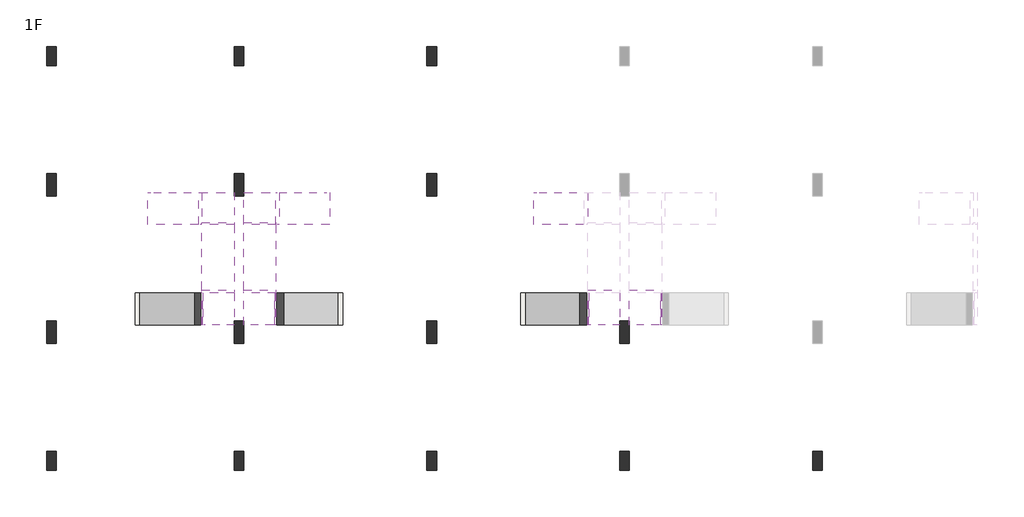
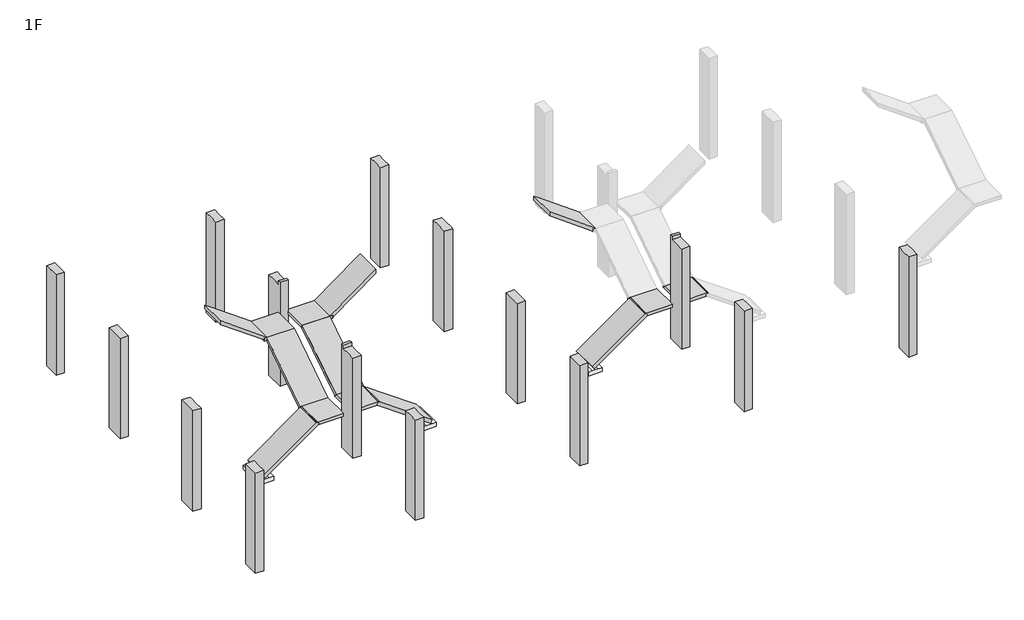
# One storey, part 1 of 2: 15 columns, 14 beams, 3 slabs.
"""IFC4 building model written with IfcOpenShell, lengths in millimetres."""

from ifc_helpers import new_model, si_unit, frame, origin, place, context, project, spatial, polyline, outline, extrude, faceted_brep, element, save

model = new_model("IFC4")

# Units and contexts
model_context = context("Model", 3, world=origin())
ifc_project = project(units=[si_unit("LENGTHUNIT", "METRE", prefix="MILLI")], contexts=[model_context])

# Site, building, storey
site = spatial("IfcSite", under=ifc_project)
building = spatial("IfcBuilding", under=site)
storey = spatial("IfcBuildingStorey", under=building, Name="1F", Elevation=30.0)

# Beams
placement = place(None, origin())
element("IfcBeam", 1, ObjectType="M_Concrete-Rectangular Beam : 1000x120", at=placement, inside=storey, context=model_context, shape_type="Brep", body=[
    faceted_brep([(4730.4772067, 5424.9999998, 1421.3386706), (4730.4772067, 4424.9999998, 1421.3386706), (4730.7175592, 4424.9999998, 1421.0), (4799.9279185, 4424.9999998, 1323.4785734), (4799.9279185, 5424.9999998, 1323.4785734), (4730.7175592, 5424.9999998, 1421.0), (2770.0, 5424.9999998, 30.0), (2839.4507118, 5424.9999998, -67.8600972), (2839.4507118, 4424.9999998, -67.8600972), (2770.0, 4424.9999998, 30.0), (4730.0, 5424.9999998, 1421.0), (4700.0000007, 5424.9999998, 1399.7091842), (4700.0000007, 4424.9999998, 1399.7091842), (4730.0, 4424.9999998, 1421.0), (4768.2542996, 4424.9999998, 1301.0), (4768.2542996, 5424.9999998, 1301.0)], [[[0, 1, 2, 3, 4, 5]], [[6, 7, 8, 9]], [[1, 0, 10, 11, 6, 9, 12, 13]], [[3, 2, 1, 13, 12, 9, 8, 14]], [[4, 3, 14, 8, 7, 15]], [[0, 5, 4, 15, 7, 6, 11, 10]]]),
])
element("IfcBeam", 2, ObjectType="M_Concrete-Rectangular Beam : 1000x120", at=placement, inside=storey, context=model_context, shape_type="Brep", body=[
    faceted_brep([(4700.0000007, 7550.0000002, 2813.0), (5700.0000007, 7550.0000002, 2813.0), (5700.0000007, 7615.755173, 2712.6194379), (4700.0000007, 7615.755173, 2712.6194379), (4700.0000007, 5424.9999998, 1421.0), (4700.0000007, 5490.7551727, 1320.6194379), (5700.0000007, 5490.7551727, 1320.6194379), (5700.0000007, 5424.9999998, 1421.0), (5700.0000007, 5524.9999998, 1343.0518141), (5700.0000007, 7585.8045224, 2693.0), (4700.0000007, 5524.9999998, 1343.0518141), (4700.0000007, 7585.8045224, 2693.0)], [[[0, 1, 2, 3]], [[4, 5, 6, 7]], [[1, 0, 4, 7]], [[2, 1, 7, 6, 8, 9]], [[3, 2, 9, 8, 6, 5, 10, 11]], [[0, 3, 11, 10, 5, 4]]]),
])
element("IfcBeam", 3, ObjectType="M_Concrete-Rectangular Beam : 1000x120", at=placement, inside=storey, context=model_context, shape_type="Brep", body=[
    faceted_brep([(4600.0000007, 7550.0000002, 2813.0), (4600.0000007, 8550.0000002, 2813.0), (4600.0000007, 8550.0000002, 2693.0), (4600.0000007, 7550.0000002, 2693.0), (5700.0000007, 8550.0000002, 2693.0), (5700.0000007, 8550.0000002, 2813.0), (5700.0000007, 7550.0000002, 2813.0), (5700.0000007, 7615.755173, 2712.6194379), (5700.0000007, 7585.8045224, 2693.0), (4700.0000007, 7550.0000002, 2813.0), (4700.0000007, 7585.8045224, 2693.0), (4700.0000007, 7550.0000002, 2693.0), (4700.0000007, 7615.755173, 2712.6194379)], [[[0, 1, 2, 3]], [[4, 5, 6, 7, 8]], [[1, 0, 9, 6, 5]], [[2, 1, 5, 4]], [[3, 2, 4, 8, 10, 11]], [[0, 3, 11, 9]], [[12, 7, 6, 9]], [[7, 12, 10, 8]], [[12, 9, 11, 10]]]),
])
element("IfcBeam", 4, ObjectType="M_Concrete-Rectangular Beam : 1000x120", at=placement, inside=storey, context=model_context, shape_type="Brep", body=[
    faceted_brep([(3020.0, 8549.9999993, 4029.9999711), (3020.0, 7549.9999993, 4029.9999711), (4699.9999533, 7549.9999993, 2813.0), (4699.9999533, 8549.9999993, 2813.0), (3199.4576422, 8549.9999993, 3900.0), (4600.0000007, 8549.9999993, 2813.0), (4600.0000007, 8549.9999993, 2737.262925), (3020.0, 8549.9999993, 3881.8224539), (3020.0, 8549.9999993, 3900.0), (3020.0, 7549.9999993, 3881.8224539), (4600.0000007, 7549.9999993, 2737.262925), (4600.0000007, 7549.9999993, 2813.0), (3020.0, 7549.9999993, 3900.0)], [[[0, 1, 2, 3, 4]], [[5, 6, 7, 8, 0, 4, 3]], [[9, 7, 6, 10]], [[10, 11, 2, 1, 12, 9]], [[1, 0, 8, 7, 9, 12]], [[5, 11, 10, 6]], [[11, 5, 3, 2]]]),
])
element("IfcBeam", 5, ObjectType="M_Concrete-Rectangular Beam : 1000x120", at=placement, inside=storey, context=model_context, shape_type="Brep", body=[
    faceted_brep([(5700.0000007, 5524.9999998, 1301.0), (4700.0000007, 5524.9999998, 1301.0), (4700.0000007, 5524.9999998, 1343.0518141), (5700.0000007, 5524.9999998, 1343.0518141), (5700.0000007, 4424.9999998, 1301.0), (5700.0000007, 4424.9999998, 1421.0), (4730.7175592, 4424.9999998, 1421.0), (4799.9279185, 4424.9999998, 1323.4785734), (4768.2542996, 4424.9999998, 1301.0), (4730.0, 4424.9999998, 1421.0), (4730.0, 5424.9999998, 1421.0), (4700.0000007, 5424.9999998, 1421.0), (4700.0000007, 4424.9999998, 1421.0), (5700.0000007, 5490.7551727, 1320.6194379), (5700.0000007, 5424.9999998, 1421.0), (4768.2542996, 5424.9999998, 1301.0), (4700.0000007, 5424.9999998, 1301.0), (4700.0000007, 5424.9999998, 1399.7091842), (4700.0000007, 4424.9999998, 1399.7091842), (4700.0000007, 5490.7551727, 1320.6194379), (4799.9279185, 5424.9999998, 1323.4785734), (4730.7175592, 5424.9999998, 1421.0)], [[[0, 1, 2, 3]], [[4, 5, 6, 7, 8]], [[9, 10, 11, 12]], [[5, 4, 0, 3, 13, 14]], [[1, 0, 4, 8, 15, 16]], [[17, 18, 12, 11, 19, 2, 1, 16]], [[20, 7, 6, 21]], [[17, 10, 9, 18]], [[7, 20, 15, 8]], [[20, 21, 10, 17, 16, 15]], [[12, 18, 9]], [[13, 19, 11, 10, 21, 14]], [[19, 13, 3, 2]], [[21, 6, 5, 14]]]),
])
element("IfcBeam", 6, ObjectType="M_Concrete-Rectangular Beam : 1000x120", at=placement, inside=storey, context=model_context, shape_type="Brep", body=[
    faceted_brep([(6969.5227948, 5424.9999998, 1421.3386706), (6969.2824423, 5424.9999998, 1421.0), (6900.0720829, 5424.9999998, 1323.4785734), (6900.0720829, 4424.9999998, 1323.4785734), (6969.2824423, 4424.9999998, 1421.0), (6969.5227948, 4424.9999998, 1421.3386706), (8930.0000014, 5424.9999998, 30.0), (8930.0000014, 4424.9999998, 30.0), (8860.5492896, 4424.9999998, -67.8600972), (8860.5492896, 5424.9999998, -67.8600972), (6970.0000014, 4424.9999998, 1421.0), (7000.0000007, 4424.9999998, 1399.7091842), (7000.0000007, 5424.9999998, 1399.7091842), (6970.0000014, 5424.9999998, 1421.0), (6931.7457019, 4424.9999998, 1301.0), (6931.7457019, 5424.9999998, 1301.0)], [[[0, 1, 2, 3, 4, 5]], [[6, 7, 8, 9]], [[5, 10, 11, 7, 6, 12, 13, 0]], [[3, 14, 8, 7, 11, 10, 5, 4]], [[2, 15, 9, 8, 14, 3]], [[0, 13, 12, 6, 9, 15, 2, 1]]]),
])
element("IfcBeam", 7, ObjectType="M_Concrete-Rectangular Beam : 1000x120", at=placement, inside=storey, context=model_context, shape_type="Brep", body=[
    faceted_brep([(7000.0000007, 7550.0000002, 2813.0), (7000.0000007, 7615.755173, 2712.6194379), (6000.0000007, 7615.755173, 2712.6194379), (6000.0000007, 7550.0000002, 2813.0), (7000.0000007, 5424.9999998, 1421.0), (6000.0000007, 5424.9999998, 1421.0), (6000.0000007, 5490.7551727, 1320.6194379), (7000.0000007, 5490.7551727, 1320.6194379), (6000.0000007, 7585.8045224, 2693.0), (6000.0000007, 5524.9999998, 1343.0518141), (7000.0000007, 7585.8045224, 2693.0), (7000.0000007, 5524.9999998, 1343.0518141)], [[[0, 1, 2, 3]], [[4, 5, 6, 7]], [[3, 5, 4, 0]], [[2, 8, 9, 6, 5, 3]], [[1, 10, 11, 7, 6, 9, 8, 2]], [[0, 4, 7, 11, 10, 1]]]),
])
element("IfcBeam", 8, ObjectType="M_Concrete-Rectangular Beam : 1000x120", at=placement, inside=storey, context=model_context, shape_type="Brep", body=[
    faceted_brep([(7100.0000007, 8550.0000002, 2813.0), (7100.0000007, 7550.0000002, 2813.0), (7100.0000007, 7550.0000002, 2693.0), (7100.0000007, 8550.0000002, 2693.0), (6000.0000007, 8550.0000002, 2813.0), (6000.0000007, 8550.0000002, 2693.0), (6000.0000007, 7585.8045224, 2693.0), (6000.0000007, 7615.755173, 2712.6194379), (6000.0000007, 7550.0000002, 2813.0), (7000.0000007, 7550.0000002, 2813.0), (7000.0000007, 7550.0000002, 2693.0), (7000.0000007, 7585.8045224, 2693.0), (7000.0000007, 7615.755173, 2712.6194379)], [[[0, 1, 2, 3]], [[4, 5, 6, 7, 8]], [[1, 0, 4, 8, 9]], [[0, 3, 5, 4]], [[3, 2, 10, 11, 6, 5]], [[2, 1, 9, 10]], [[12, 9, 8, 7]], [[12, 7, 6, 11]], [[9, 12, 11, 10]]]),
])
element("IfcBeam", 9, ObjectType="M_Concrete-Rectangular Beam : 1000x120", at=placement, inside=storey, context=model_context, shape_type="Brep", body=[
    faceted_brep([(7000.0000481, 8549.9999993, 2813.0), (7000.0000481, 7549.9999993, 2813.0), (8680.0000414, 7549.9999993, 4030.0), (8680.0, 8549.9999993, 4029.99997), (8500.5423593, 8549.9999993, 3900.0), (7100.0000007, 8549.9999993, 2737.262925), (7100.0000007, 8549.9999993, 2813.0), (8680.0, 8549.9999993, 3900.0), (8680.0, 8549.9999993, 3881.8224529), (7100.0000007, 7549.9999993, 2737.262925), (8680.0, 7549.9999993, 3881.8224529), (7100.0000007, 7549.9999993, 2813.0), (8680.0, 7549.9999993, 3900.0)], [[[0, 1, 2, 3, 4]], [[5, 6, 0, 4, 3, 7, 8]], [[9, 5, 8, 10]], [[11, 9, 10, 12, 2, 1]], [[11, 6, 5, 9]], [[6, 11, 1, 0]], [[3, 2, 12, 10, 8, 7]]]),
])
element("IfcBeam", 10, ObjectType="M_Concrete-Rectangular Beam : 1000x120", at=placement, inside=storey, context=model_context, shape_type="Brep", body=[
    faceted_brep([(7000.0000007, 5524.9999998, 1301.0), (6000.0000007, 5524.9999998, 1301.0), (6000.0000007, 5524.9999998, 1343.0518141), (7000.0000007, 5524.9999998, 1343.0518141), (6000.0000007, 4424.9999998, 1421.0), (6000.0000007, 4424.9999998, 1301.0), (6931.7457019, 4424.9999998, 1301.0), (6900.0720829, 4424.9999998, 1323.4785734), (6969.2824423, 4424.9999998, 1421.0), (6970.0000014, 5424.9999998, 1421.0), (6970.0000014, 4424.9999998, 1421.0), (7000.0000007, 4424.9999998, 1421.0), (7000.0000007, 5424.9999998, 1421.0), (6000.0000007, 5424.9999998, 1421.0), (6000.0000007, 5490.7551727, 1320.6194379), (7000.0000007, 5424.9999998, 1301.0), (6931.7457019, 5424.9999998, 1301.0), (7000.0000007, 4424.9999998, 1399.7091842), (7000.0000007, 5424.9999998, 1399.7091842), (7000.0000007, 5490.7551727, 1320.6194379), (6900.0720829, 5424.9999998, 1323.4785734), (6969.2824423, 5424.9999998, 1421.0)], [[[0, 1, 2, 3]], [[4, 5, 6, 7, 8]], [[9, 10, 11, 12]], [[5, 4, 13, 14, 2, 1]], [[1, 0, 15, 16, 6, 5]], [[17, 18, 15, 0, 3, 19, 12, 11]], [[7, 20, 21, 8]], [[10, 9, 18, 17]], [[20, 7, 6, 16]], [[21, 20, 16, 15, 18, 9]], [[17, 11, 10]], [[19, 14, 13, 21, 9, 12]], [[14, 19, 3, 2]], [[8, 21, 13, 4]]]),
])
element("IfcBeam", 11, ObjectType="M_Concrete-Rectangular Beam : 1000x120", at=placement, inside=storey, context=model_context, shape_type="Brep", body=[
    faceted_brep([(16730.4772117, 5424.9999998, 1421.3386706), (16730.4772117, 4424.9999998, 1421.3386706), (16730.7175642, 4424.9999998, 1421.0), (16799.9279236, 4424.9999998, 1323.4785734), (16799.9279236, 5424.9999998, 1323.4785734), (16730.7175642, 5424.9999998, 1421.0), (14770.000005, 5424.9999998, 30.0), (14839.4507169, 5424.9999998, -67.8600972), (14839.4507169, 4424.9999998, -67.8600972), (14770.000005, 4424.9999998, 30.0), (16730.000005, 5424.9999998, 1421.0), (16700.0000058, 5424.9999998, 1399.7091842), (16700.0000058, 4424.9999998, 1399.7091842), (16730.000005, 4424.9999998, 1421.0), (16768.2543046, 4424.9999998, 1301.0), (16768.2543046, 5424.9999998, 1301.0)], [[[0, 1, 2, 3, 4, 5]], [[6, 7, 8, 9]], [[1, 0, 10, 11, 6, 9, 12, 13]], [[3, 2, 1, 13, 12, 9, 8, 14]], [[4, 3, 14, 8, 7, 15]], [[0, 5, 4, 15, 7, 6, 11, 10]]]),
])
element("IfcBeam", 12, ObjectType="M_Concrete-Rectangular Beam : 1000x120", at=placement, inside=storey, context=model_context, shape_type="Brep", body=[
    faceted_brep([(16699.9999584, 7549.9999993, 2813.0), (16699.9999584, 8549.9999993, 2813.0), (15199.4576472, 8549.9999993, 3900.0), (15019.9999651, 8549.9999993, 4030.0), (15020.0000057, 7549.9999993, 4029.9999706), (16600.0000058, 8549.9999993, 2813.0), (16600.0000058, 8549.9999993, 2737.262925), (15020.0000057, 8549.9999993, 3881.8224534), (15020.0000057, 8549.9999993, 3900.0), (16600.0000058, 7549.9999993, 2737.262925), (15020.0000057, 7549.9999993, 3881.8224534), (16600.0000058, 7549.9999993, 2813.0), (15020.0000057, 7549.9999993, 3900.0)], [[[0, 1, 2, 3, 4]], [[5, 6, 7, 8, 3, 2, 1]], [[6, 9, 10, 7]], [[9, 11, 0, 4, 12, 10]], [[5, 11, 9, 6]], [[11, 5, 1, 0]], [[4, 3, 8, 7, 10, 12]]]),
])
element("IfcBeam", 13, ObjectType="M_Concrete-Rectangular Beam : 1000x120", at=placement, inside=storey, context=model_context, shape_type="Brep", body=[
    faceted_brep([(17700.0000058, 5524.9999998, 1301.0), (16700.0000058, 5524.9999998, 1301.0), (16700.0000058, 5524.9999998, 1343.0518141), (17700.0000058, 5524.9999998, 1343.0518141), (17700.0000058, 4424.9999998, 1301.0), (17700.0000058, 4424.9999998, 1421.0), (16730.7175642, 4424.9999998, 1421.0), (16799.9279236, 4424.9999998, 1323.4785734), (16768.2543046, 4424.9999998, 1301.0), (16730.000005, 4424.9999998, 1421.0), (16730.000005, 5424.9999998, 1421.0), (16700.0000058, 5424.9999998, 1421.0), (16700.0000058, 4424.9999998, 1421.0), (17700.0000058, 5490.7551727, 1320.6194379), (17700.0000058, 5424.9999998, 1421.0), (16768.2543046, 5424.9999998, 1301.0), (16700.0000058, 5424.9999998, 1301.0), (16700.0000058, 5424.9999998, 1399.7091842), (16700.0000058, 4424.9999998, 1399.7091842), (16700.0000058, 5490.7551727, 1320.6194379), (16799.9279236, 5424.9999998, 1323.4785734), (16730.7175642, 5424.9999998, 1421.0)], [[[0, 1, 2, 3]], [[4, 5, 6, 7, 8]], [[9, 10, 11, 12]], [[5, 4, 0, 3, 13, 14]], [[1, 0, 4, 8, 15, 16]], [[17, 18, 12, 11, 19, 2, 1, 16]], [[20, 7, 6, 21]], [[17, 10, 9, 18]], [[7, 20, 15, 8]], [[20, 21, 10, 17, 16, 15]], [[12, 18, 9]], [[13, 19, 11, 10, 21, 14]], [[19, 13, 3, 2]], [[21, 6, 5, 14]]]),
])
element("IfcBeam", 14, ObjectType="M_Concrete-Rectangular Beam : 1000x120", at=placement, inside=storey, context=model_context, shape_type="Brep", body=[
    faceted_brep([(19000.0000058, 5524.9999998, 1301.0), (18000.0000058, 5524.9999998, 1301.0), (18000.0000058, 5524.9999998, 1343.0518141), (19000.0000058, 5524.9999998, 1343.0518141), (18000.0000058, 4424.9999998, 1421.0), (18000.0000058, 4424.9999998, 1301.0), (18931.7457069, 4424.9999998, 1301.0), (18900.072088, 4424.9999998, 1323.4785734), (18969.2824473, 4424.9999998, 1421.0), (18970.0000065, 5424.9999998, 1421.0), (18970.0000065, 4424.9999998, 1421.0), (19000.0000058, 4424.9999998, 1421.0), (19000.0000058, 5424.9999998, 1421.0), (18000.0000058, 5424.9999998, 1421.0), (18000.0000058, 5490.7551727, 1320.6194379), (19000.0000058, 5424.9999998, 1301.0), (18931.7457069, 5424.9999998, 1301.0), (19000.0000058, 4424.9999998, 1399.7091842), (19000.0000058, 5424.9999998, 1399.7091842), (19000.0000058, 5490.7551727, 1320.6194379), (18900.072088, 5424.9999998, 1323.4785734), (18969.2824473, 5424.9999998, 1421.0)], [[[0, 1, 2, 3]], [[4, 5, 6, 7, 8]], [[9, 10, 11, 12]], [[5, 4, 13, 14, 2, 1]], [[1, 0, 15, 16, 6, 5]], [[17, 18, 15, 0, 3, 19, 12, 11]], [[7, 20, 21, 8]], [[10, 9, 18, 17]], [[20, 7, 6, 16]], [[21, 20, 16, 15, 18, 9]], [[17, 11, 10]], [[19, 14, 13, 21, 9, 12]], [[14, 19, 3, 2]], [[8, 21, 13, 4]]]),
])

# Columns
element("IfcColumn", 15, ObjectType="M_Concrete-Rectangular-Column : 300x600", at=placement, inside=storey, context=model_context, shape_type="Brep", body=[
    faceted_brep([(165.0, 499.9999998, 30.0), (165.0, -100.0000002, 30.0), (-135.0, -100.0000002, 30.0), (-135.0, 499.9999998, 30.0), (165.0, 499.9999998, 3630.0), (165.0, 499.9999998, 3900.0), (165.0, 200.000001, 3900.0), (165.0, -100.0000002, 3900.0), (165.0, -100.0000002, 3330.0), (-135.0, -100.0000002, 3900.0), (-135.0, -100.0000002, 3330.0), (-135.0, 499.9999998, 3900.0), (-135.0, 499.9999998, 3630.0)], [[[0, 1, 2, 3]], [[1, 0, 4, 5, 6, 7, 8]], [[2, 1, 8, 7, 9, 10]], [[3, 2, 10, 9, 11, 12]], [[0, 3, 12, 11, 5, 4]], [[7, 6, 5, 11, 9]]]),
])
element("IfcColumn", 16, ObjectType="M_Concrete-Rectangular-Column : 300x600", at=placement, inside=storey, context=model_context, shape_type="Brep", body=[
    faceted_brep([(164.9999993, 13100.0000003, 30.0), (164.9999993, 12500.0000003, 30.0), (-135.0000007, 12500.0000003, 30.0), (-135.0000007, 13100.0000003, 30.0), (164.9999993, 13100.0000003, 3330.0), (164.9999993, 13100.0000003, 3900.0), (164.9999993, 12799.9999993, 3900.0), (164.9999993, 12500.0000003, 3900.0), (-135.0000007, 12500.0000003, 3900.0), (-135.0000007, 13100.0000003, 3900.0)], [[[0, 1, 2, 3]], [[1, 0, 4, 5, 6, 7]], [[2, 1, 7, 8]], [[3, 2, 8, 9]], [[0, 3, 9, 5, 4]], [[7, 6, 5, 9, 8]]]),
])
element("IfcColumn", 17, ObjectType="M_Concrete-Rectangular-Column : 300x600", at=placement, inside=storey, context=model_context, shape_type="Brep", body=[
    faceted_brep([(6000.0000007, 499.9999998, 30.0), (6000.0000007, -100.0000002, 30.0), (5700.0000007, -100.0000002, 30.0), (5700.0000007, 499.9999998, 30.0), (6000.0000007, 499.9999998, 3630.0), (6000.0000007, 499.9999998, 3900.0), (6000.0000007, 200.000001, 3900.0), (6000.0000007, -100.0000002, 3900.0), (6000.0000007, -100.0000002, 3330.0), (5700.0000007, -100.0000002, 3900.0), (5700.0000007, -100.0000002, 3330.0), (5700.0000007, 200.000001, 3900.0), (5700.0000007, 499.9999998, 3900.0), (5700.0000007, 499.9999998, 3630.0)], [[[0, 1, 2, 3]], [[1, 0, 4, 5, 6, 7, 8]], [[2, 1, 8, 7, 9, 10]], [[3, 2, 10, 9, 11, 12, 13]], [[0, 3, 13, 12, 5, 4]], [[7, 6, 5, 12, 11, 9]]]),
])
element("IfcColumn", 18, ObjectType="M_Concrete-Rectangular-Column : 300x600", at=placement, inside=storey, context=model_context, shape_type="Brep", body=[
    faceted_brep([(12000.0000034, 499.9999998, 30.0), (12000.0000034, -100.0000002, 30.0), (11700.0000034, -100.0000002, 30.0), (11700.0000034, 499.9999998, 30.0), (12000.0000034, 499.9999998, 3630.0), (12000.0000034, 499.9999998, 3900.0), (12000.0000034, 200.000001, 3900.0), (12000.0000034, -100.0000002, 3900.0), (12000.0000034, -100.0000002, 3330.0), (11700.0000034, -100.0000002, 3900.0), (11700.0000034, -100.0000002, 3330.0), (11700.0000034, 200.000001, 3900.0), (11700.0000034, 499.9999998, 3900.0), (11700.0000034, 499.9999998, 3630.0)], [[[0, 1, 2, 3]], [[1, 0, 4, 5, 6, 7, 8]], [[2, 1, 8, 7, 9, 10]], [[3, 2, 10, 9, 11, 12, 13]], [[0, 3, 13, 12, 5, 4]], [[7, 6, 5, 12, 11, 9]]]),
])
element("IfcColumn", 19, ObjectType="M_Concrete-Rectangular-Column : 300x600", at=placement, inside=storey, context=model_context, shape_type="Brep", body=[
    faceted_brep([(18000.0000058, 499.9999998, 30.0), (18000.0000058, -100.0000002, 30.0), (17700.0000058, -100.0000002, 30.0), (17700.0000058, 499.9999998, 30.0), (18000.0000058, 499.9999998, 3900.0), (18000.0000058, 200.000001, 3900.0), (18000.0000058, -100.0000002, 3900.0), (17700.0000058, -100.0000002, 3900.0), (17700.0000058, -100.0000002, 3330.0), (17700.0000058, 200.000001, 3900.0), (17700.0000058, 499.9999998, 3900.0)], [[[0, 1, 2, 3]], [[1, 0, 4, 5, 6]], [[2, 1, 6, 7, 8]], [[3, 2, 8, 7, 9, 10]], [[0, 3, 10, 4]], [[6, 5, 4, 10, 9, 7]]]),
])
element("IfcColumn", 20, ObjectType="M_Concrete-Rectangular-Column : 300x600", at=placement, inside=storey, context=model_context, shape_type="Brep", body=[
    faceted_brep([(24000.0000047, 499.9999998, 30.0), (24000.0000047, -100.0000002, 30.0), (23700.0000047, -100.0000002, 30.0), (23700.0000047, 499.9999998, 30.0), (24000.0000047, 499.9999998, 3900.0), (24000.0000047, 200.000001, 3900.0), (24000.0000047, -100.0000002, 3900.0), (23700.0000047, -100.0000002, 3900.0), (23700.0000047, -100.0000002, 3330.0), (23700.0000047, 200.000001, 3900.0), (23700.0000047, 499.9999998, 3900.0)], [[[0, 1, 2, 3]], [[1, 0, 4, 5, 6]], [[2, 1, 6, 7, 8]], [[3, 2, 8, 7, 9, 10]], [[0, 3, 10, 4]], [[6, 5, 4, 10, 9, 7]]]),
])
element("IfcColumn", 21, ObjectType="M_Concrete-Rectangular-Column : 300x600", at=placement, inside=storey, context=model_context, shape_type="Brep", body=[
    faceted_brep([(6000.0000007, 13100.0000003, 30.0), (6000.0000007, 12500.0000003, 30.0), (5700.0000007, 12500.0000003, 30.0), (5700.0000007, 13100.0000003, 30.0), (6000.0000007, 13100.0000003, 3330.0), (6000.0000007, 13100.0000003, 3900.0), (6000.0000007, 12799.9999993, 3900.0), (6000.0000007, 12500.0000003, 3900.0), (6000.0000007, 12500.0000003, 3630.0), (5700.0000007, 12500.0000003, 3900.0), (5700.0000007, 12500.0000003, 3630.0), (5700.0000007, 12799.9999993, 3900.0), (5700.0000007, 13100.0000003, 3900.0), (5700.0000007, 13100.0000003, 3330.0)], [[[0, 1, 2, 3]], [[1, 0, 4, 5, 6, 7, 8]], [[2, 1, 8, 7, 9, 10]], [[3, 2, 10, 9, 11, 12, 13]], [[0, 3, 13, 12, 5, 4]], [[7, 6, 5, 12, 11, 9]]]),
])
element("IfcColumn", 22, ObjectType="M_Concrete-Rectangular-Column : 300x600", at=placement, inside=storey, context=model_context, shape_type="Brep", body=[
    faceted_brep([(12000.0000034, 13100.0000003, 30.0), (12000.0000034, 12500.0000003, 30.0), (11700.0000034, 12500.0000003, 30.0), (11700.0000034, 13100.0000003, 30.0), (12000.0000034, 13100.0000003, 3330.0), (12000.0000034, 13100.0000003, 3900.0), (12000.0000034, 12799.9999993, 3900.0), (12000.0000034, 12500.0000003, 3900.0), (12000.0000034, 12500.0000003, 3630.0), (11700.0000034, 12500.0000003, 3900.0), (11700.0000034, 12500.0000003, 3630.0), (11700.0000034, 12799.9999993, 3900.0), (11700.0000034, 13100.0000003, 3900.0), (11700.0000034, 13100.0000003, 3330.0)], [[[0, 1, 2, 3]], [[1, 0, 4, 5, 6, 7, 8]], [[2, 1, 8, 7, 9, 10]], [[3, 2, 10, 9, 11, 12, 13]], [[0, 3, 13, 12, 5, 4]], [[7, 6, 5, 12, 11, 9]]]),
])
element("IfcColumn", 23, ObjectType="M_Concrete-Rectangular-Column : 300x700", at=placement, inside=storey, context=model_context, shape_type="Brep", body=[
    faceted_brep([(165.0, 4550.0000002, 30.0), (165.0, 3850.0000002, 30.0), (-135.0, 3850.0000002, 30.0), (-135.0, 4550.0000002, 30.0), (165.0, 4550.0000002, 3630.0), (165.0, 4550.0000002, 3900.0), (165.0, 4449.9999998, 3900.0), (165.0, 4149.9999998, 3900.0), (165.0, 3850.0000002, 3900.0), (165.0, 3850.0000002, 3630.0), (-135.0, 3850.0000002, 3900.0), (-135.0, 3850.0000002, 3630.0), (-135.0, 4550.0000002, 3900.0), (-135.0, 4550.0000002, 3630.0)], [[[0, 1, 2, 3]], [[1, 0, 4, 5, 6, 7, 8, 9]], [[2, 1, 9, 8, 10, 11]], [[3, 2, 11, 10, 12, 13]], [[0, 3, 13, 12, 5, 4]], [[8, 7, 6, 5, 12, 10]]]),
])
element("IfcColumn", 24, ObjectType="M_Concrete-Rectangular-Column : 300x700", at=placement, inside=storey, context=model_context, shape_type="Brep", body=[
    faceted_brep([(165.0, 9149.9985388, 30.0), (165.0, 8449.9985388, 30.0), (-135.0, 8449.9985388, 30.0), (-135.0, 9149.9985388, 30.0), (165.0, 9149.9985388, 3630.0), (165.0, 9149.9985388, 3900.0), (165.0, 8849.9999993, 3900.0), (165.0, 8549.9999993, 3900.0), (165.0, 8449.9985388, 3900.0), (165.0, 8449.9985388, 3630.0), (-135.0, 8449.9985388, 3900.0), (-135.0, 8449.9985388, 3630.0), (-135.0, 9149.9985388, 3900.0), (-135.0, 9149.9985388, 3630.0)], [[[0, 1, 2, 3]], [[1, 0, 4, 5, 6, 7, 8, 9]], [[2, 1, 9, 8, 10, 11]], [[3, 2, 11, 10, 12, 13]], [[0, 3, 13, 12, 5, 4]], [[8, 7, 6, 5, 12, 10]]]),
])
element("IfcColumn", 25, ObjectType="M_Concrete-Rectangular-Column : 300x700", at=placement, inside=storey, context=model_context, shape_type="Brep", body=[
    faceted_brep([(6000.0000007, 4550.0000002, 30.0), (6000.0000007, 3850.0000002, 30.0), (5700.0000007, 3850.0000002, 30.0), (5700.0000007, 4550.0000002, 30.0), (6000.0000007, 4550.0000002, 4030.0), (6000.0000007, 4450.0000002, 4030.0), (6000.0000007, 4450.0000002, 3900.0), (6000.0000007, 4149.9999998, 3900.0), (6000.0000007, 3850.0000002, 3900.0), (6000.0000007, 3850.0000002, 3630.0), (5700.0000007, 3850.0000002, 3900.0), (5700.0000007, 3850.0000002, 3630.0), (5700.0000007, 4149.9999998, 3900.0), (5700.0000007, 4450.0000002, 3900.0), (5700.0000007, 4450.0000002, 4030.0), (5700.0000007, 4550.0000002, 4030.0)], [[[0, 1, 2, 3]], [[1, 0, 4, 5, 6, 7, 8, 9]], [[2, 1, 9, 8, 10, 11]], [[3, 2, 11, 10, 12, 13, 14, 15]], [[0, 3, 15, 4]], [[4, 15, 14, 5]], [[6, 13, 12, 10, 8, 7]], [[13, 6, 5, 14]]]),
])
element("IfcColumn", 26, ObjectType="M_Concrete-Rectangular-Column : 300x700", at=placement, inside=storey, context=model_context, shape_type="Brep", body=[
    faceted_brep([(12000.0000034, 4550.0000002, 30.0), (12000.0000034, 3850.0000002, 30.0), (11700.0000034, 3850.0000002, 30.0), (11700.0000034, 4550.0000002, 30.0), (12000.0000034, 4550.0000002, 3900.0), (12000.0000034, 4449.9999998, 3900.0), (12000.0000034, 4149.9999998, 3900.0), (12000.0000034, 3850.0000002, 3900.0), (12000.0000034, 3850.0000002, 3630.0), (11700.0000034, 3850.0000002, 3900.0), (11700.0000034, 3850.0000002, 3630.0), (11700.0000034, 4149.9999998, 3900.0), (11700.0000034, 4449.9999998, 3900.0), (11700.0000034, 4550.0000002, 3900.0)], [[[0, 1, 2, 3]], [[1, 0, 4, 5, 6, 7, 8]], [[2, 1, 8, 7, 9, 10]], [[3, 2, 10, 9, 11, 12, 13]], [[0, 3, 13, 4]], [[7, 6, 5, 4, 13, 12, 11, 9]]]),
])
element("IfcColumn", 27, ObjectType="M_Concrete-Rectangular-Column : 300x700", at=placement, inside=storey, context=model_context, shape_type="Brep", body=[
    faceted_brep([(18000.0000058, 4550.0000002, 30.0), (18000.0000058, 3850.0000002, 30.0), (17700.0000058, 3850.0000002, 30.0), (17700.0000058, 4550.0000002, 30.0), (18000.0000058, 4550.0000002, 4030.0), (18000.0000058, 4450.0000002, 4030.0), (18000.0000058, 4450.0000002, 3900.0), (18000.0000058, 4149.9999998, 3900.0), (18000.0000058, 3850.0000002, 3900.0), (17700.0000058, 3850.0000002, 3900.0), (17700.0000058, 4149.9999998, 3900.0), (17700.0000058, 4450.0000002, 3900.0), (17700.0000058, 4450.0000002, 4030.0), (17700.0000058, 4550.0000002, 4030.0)], [[[0, 1, 2, 3]], [[1, 0, 4, 5, 6, 7, 8]], [[2, 1, 8, 9]], [[3, 2, 9, 10, 11, 12, 13]], [[0, 3, 13, 4]], [[4, 13, 12, 5]], [[6, 11, 10, 9, 8, 7]], [[11, 6, 5, 12]]]),
])
element("IfcColumn", 28, ObjectType="M_Concrete-Rectangular-Column : 300x700", at=placement, inside=storey, context=model_context, shape_type="Brep", body=[
    faceted_brep([(6000.0000007, 9149.9985388, 30.0), (6000.0000007, 8449.9985388, 30.0), (5700.0000007, 8449.9985388, 30.0), (5700.0000007, 9149.9985388, 30.0), (6000.0000007, 9149.9985388, 3630.0), (6000.0000007, 9149.9985388, 3900.0), (6000.0000007, 8849.9999993, 3900.0), (6000.0000007, 8549.9999993, 3900.0), (6000.0000007, 8549.9999993, 4030.0), (6000.0000007, 8449.9985388, 4030.0), (5700.0000007, 8449.9985388, 4030.0), (5700.0000007, 8549.9999993, 4030.0), (5700.0000007, 8549.9999993, 3900.0), (5700.0000007, 8849.9999993, 3900.0), (5700.0000007, 9149.9985388, 3900.0), (5700.0000007, 9149.9985388, 3630.0)], [[[0, 1, 2, 3]], [[1, 0, 4, 5, 6, 7, 8, 9]], [[2, 1, 9, 10]], [[3, 2, 10, 11, 12, 13, 14, 15]], [[0, 3, 15, 14, 5, 4]], [[10, 9, 8, 11]], [[12, 7, 6, 5, 14, 13]], [[7, 12, 11, 8]]]),
])
element("IfcColumn", 29, ObjectType="M_Concrete-Rectangular-Column : 300x700", at=placement, inside=storey, context=model_context, shape_type="Brep", body=[
    faceted_brep([(12000.0000034, 9149.9985388, 30.0), (12000.0000034, 8449.9985388, 30.0), (11700.0000034, 8449.9985388, 30.0), (11700.0000034, 9149.9985388, 30.0), (12000.0000034, 9149.9985388, 3630.0), (12000.0000034, 9149.9985388, 3900.0), (12000.0000034, 8849.9999993, 3900.0), (12000.0000034, 8549.9999993, 3900.0), (12000.0000034, 8449.9985388, 3900.0), (11700.0000034, 8449.9985388, 3900.0), (11700.0000034, 8549.9999993, 3900.0), (11700.0000034, 8849.9999993, 3900.0), (11700.0000034, 9149.9985388, 3900.0), (11700.0000034, 9149.9985388, 3630.0)], [[[0, 1, 2, 3]], [[1, 0, 4, 5, 6, 7, 8]], [[2, 1, 8, 9]], [[3, 2, 9, 10, 11, 12, 13]], [[0, 3, 13, 12, 5, 4]], [[8, 7, 6, 5, 12, 11, 10, 9]]]),
])

# Slabs
element("IfcSlab", 30, ObjectType="Mong bang-lech tam : 520x300", at=placement, inside=storey, context=model_context, shape_type="SweptSolid", body=[
    extrude(outline(polyline([(-120.0, 2770.0), (-120.0, 2620.0), (-270.0, 2620.0), (-270.0, 3140.0), (-120.0, 3140.0), (-120.0, 2990.0), (-120.0, 2770.0)])), frame((0.0, 4424.9999998, 0.0), z_axis=(0.0, 1.0, 0.0), x_axis=(0.0, 0.0, 1.0)), (0.0, 0.0, 1.0), 1000.0),
])
element("IfcSlab", 31, ObjectType="Mong bang-lech tam : 520x300", at=placement, inside=storey, context=model_context, shape_type="SweptSolid", body=[
    extrude(outline(polyline([(-120.0, 8930.0000014), (-120.0, 8710.0000014), (-120.0, 8560.0000014), (-270.0, 8560.0000014), (-270.0, 9080.0000014), (-120.0, 9080.0000014), (-120.0, 8930.0000014)])), frame((0.0, 4424.9999998, 0.0), z_axis=(0.0, 1.0, 0.0), x_axis=(0.0, 0.0, 1.0)), (0.0, 0.0, 1.0), 1000.0),
])
element("IfcSlab", 32, ObjectType="Mong bang-lech tam : 520x300", at=placement, inside=storey, context=model_context, shape_type="SweptSolid", body=[
    extrude(outline(polyline([(-120.0, 14770.000005), (-120.0, 14620.000005), (-270.0, 14620.000005), (-270.0, 15140.000005), (-120.0, 15140.000005), (-120.0, 14990.000005), (-120.0, 14770.000005)])), frame((0.0, 4424.9999998, 0.0), z_axis=(0.0, 1.0, 0.0), x_axis=(0.0, 0.0, 1.0)), (0.0, 0.0, 1.0), 1000.0),
])

save(model, "model.ifc")

# Revit data of these elements
# Type "M_Concrete-Rectangular Beam : 1000x120"
#   Length [instance default] = 1524 mm
#   b = 1000 mm
#   h = 120 mm
#   Structural Material [instance default] = Concrete, Cast-in-Place gray
#   Assembly Code = ""
# Type "M_Concrete-Rectangular-Column : 300x600"
#   b = 300 mm
#   h = 600 mm
#   Structural Material [instance default] = Concrete, Cast-in-Place gray
# Type "M_Concrete-Rectangular-Column : 300x700"
#   b = 300 mm
#   h = 700 mm
#   Structural Material [instance default] = Concrete, Cast-in-Place gray
# Type "Mong bang-lech tam : 520x300"
#   Length = 1000 mm
#   Lech Tam (E) = 0 mm
#   Foundation Thickness = 150 mm
#   Foundation (h2) = 150 mm
#   Foundation (h1) = 0 mm
#   Be Rong Dam (b) = 220 mm
#   Be Rong Dai Mong (B) = 520 mm
#   Structural Material [instance default] = Concrete, Cast-in-Place gray
#   Width = 0
#   Assembly Code = ""
# Elements 1, 6, 11 (IfcBeam, "M_Concrete-Rectangular Beam : 1000x120")
#   Comments = ""
#   COF_GEN__Name = "STAIR"
#   Structural Material = Concrete, Cast-in-Place gray
#   Phase Created = New Construction
#   Materials on its faces: "Concrete, Cast-in-Place gray"
# Elements 2, 3, 4, 5, 7, 8, 9, 10, 12, 13, 14 (IfcBeam, "M_Concrete-Rectangular Beam : 1000x120")
#   COF_GEN__Name = "STAIR"
#   Structural Material = Concrete, Cast-in-Place gray
#   Phase Created = New Construction
#   Materials on its faces: "Concrete, Cast-in-Place gray"
# Elements 15, 16, 17, 18, 20, 21, 22 (IfcColumn, "M_Concrete-Rectangular-Column : 300x600")
#   Comments = ""
#   COF_CON__WorkItemNumber = "SH3-A-02F"
#   COF_GEN__Name = "C1"
#   Structural Material = Concrete, Cast-in-Place gray
#   Phase Created = New Construction
#   Materials on its faces: "Concrete, Cast-in-Place gray"
# Element 19 (IfcColumn, "M_Concrete-Rectangular-Column : 300x600")
#   Comments = ""
#   COF_CON__WorkItemNumber = "SH3-A-02F"
#   COF_GEN__Name = "C2"
#   Structural Material = Concrete, Cast-in-Place gray
#   Phase Created = New Construction
#   Materials on its faces: "Concrete, Cast-in-Place gray"
# Elements 23, 24 (IfcColumn, "M_Concrete-Rectangular-Column : 300x700")
#   Comments = ""
#   COF_CON__WorkItemNumber = "SH3-A-02F"
#   COF_GEN__Name = "C3"
#   Structural Material = Concrete, Cast-in-Place gray
#   Phase Created = New Construction
#   Materials on its faces: "Concrete, Cast-in-Place gray"
# Elements 25, 28 (IfcColumn, "M_Concrete-Rectangular-Column : 300x700")
#   Comments = ""
#   COF_CON__WorkItemNumber = "SH3-A-02F"
#   COF_GEN__Name = "C4"
#   Structural Material = Concrete, Cast-in-Place gray
#   Phase Created = New Construction
#   Materials on its faces: "Concrete, Cast-in-Place gray"
# Elements 26, 29 (IfcColumn, "M_Concrete-Rectangular-Column : 300x700")
#   Comments = ""
#   COF_CON__WorkItemNumber = "SH3-A-02F"
#   COF_GEN__Name = "C5"
#   Structural Material = Concrete, Cast-in-Place gray
#   Phase Created = New Construction
#   Materials on its faces: "Concrete, Cast-in-Place gray"
# Element 27 (IfcColumn, "M_Concrete-Rectangular-Column : 300x700")
#   Comments = ""
#   COF_CON__WorkItemNumber = "SH3-A-02F"
#   COF_GEN__Name = "C6"
#   Structural Material = Concrete, Cast-in-Place gray
#   Phase Created = New Construction
#   Materials on its faces: "Concrete, Cast-in-Place gray"
# Elements 30, 31, 32 (IfcSlab, "Mong bang-lech tam : 520x300")
#   Comments = ""
#   COF_GEN__Name = "DCT"
#   Structural Material = Concrete, Cast-in-Place gray
#   Phase Created = New Construction
#   Materials on its faces: "Concrete, Cast-in-Place gray"
# Materials
#   "Concrete, Cast-in-Place gray": class "Concrete", colour RGB 207 208 204, transparency 0, Description = "Cast-in-place concrete", Cost = 0
